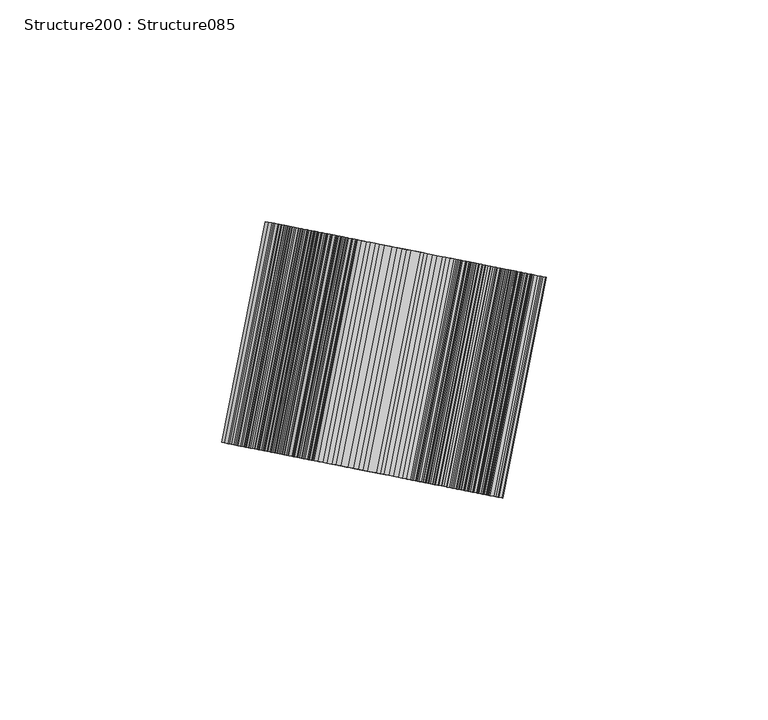
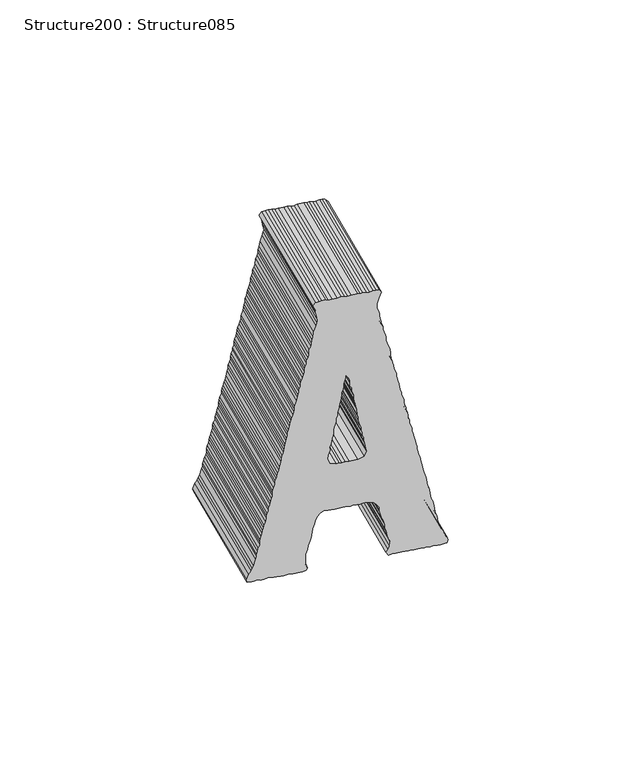
"""IFC4 building model written with IfcOpenShell, lengths in millimetres: proxy geometry, Structure200 : Structure085."""

import ifcopenshell
import ifcopenshell.guid

model = None  # the IFC model being written
_history = None  # IfcOwnerHistory: only IFC2X3 demands one
_inside = {}  # id of a spatial element -> (the spatial element, [elements in it])
_under = {}  # id of a project, library or spatial element -> (it, [spatial elements below it])
_declared = {}  # id of a project -> (the project, [libraries it declares])
_typed = {}  # id of a type object -> (the type object, [elements of that type])
_made_of = {}  # id of a material, layer set ... -> (it, [elements and type objects made of it])


def new_model(schema):
    """Start an empty IFC model of exactly this schema.

    Asked for "IFC4X3", IfcOpenShell would pick the latest addendum, in which some entities
    have other attributes; the version numbers below select the first issue.
    IFC2X3 requires an IfcOwnerHistory on every rooted entity: one is made here for all.
    """
    global model, _history
    if schema == "IFC4X3":
        model = ifcopenshell.file(schema_version=(4, 3, 0, 0))
    else:
        model = ifcopenshell.file(schema=schema)
    _inside.clear()
    _under.clear()
    _declared.clear()
    _typed.clear()
    _made_of.clear()
    _history = None
    if model.schema == "IFC2X3":
        org = make("IfcOrganization", Name="unknown")
        user = make(
            "IfcPersonAndOrganization",
            ThePerson=make("IfcPerson", FamilyName="unknown"),
            TheOrganization=org,
        )
        app = make(
            "IfcApplication",
            ApplicationDeveloper=org,
            Version="unknown",
            ApplicationFullName="unknown",
            ApplicationIdentifier="unknown",
        )
        _history = make(
            "IfcOwnerHistory",
            OwningUser=user,
            OwningApplication=app,
            ChangeAction="ADDED",
            CreationDate=0,
        )
    return model


def make(cls, **values):
    """One entity of the class cls with the attributes given. An attribute that is None is left unset."""
    return model.create_entity(
        cls, **{name: value for name, value in values.items() if value is not None}
    )


def rooted(cls, **values):
    """An entity with a GlobalId (a new one), such as an element, a storey or a relation."""
    return make(cls, GlobalId=ifcopenshell.guid.new(), OwnerHistory=_history, **values)


def si_unit(unit_type, name, prefix=None):
    """IfcSIUnit, for example si_unit("LENGTHUNIT", "METRE", prefix="MILLI")."""
    return make("IfcSIUnit", UnitType=unit_type, Prefix=prefix, Name=name)


def assignment(units):
    """IfcUnitAssignment: the units of a project."""
    return None if units is None else make("IfcUnitAssignment", Units=units)


def point(xyz):
    """IfcCartesianPoint."""
    return None if xyz is None else make("IfcCartesianPoint", Coordinates=xyz)


def direction(xyz):
    """IfcDirection."""
    return None if xyz is None else make("IfcDirection", DirectionRatios=xyz)


def frame(location, z_axis=None, x_axis=None):
    """IfcAxis2Placement3D, a coordinate frame: its origin and axes. An axis left out is left unset."""
    return make(
        "IfcAxis2Placement3D",
        Location=point(location),
        Axis=direction(z_axis),
        RefDirection=direction(x_axis),
    )


def origin():
    """The frame at (0, 0, 0) with its axes left unset."""
    return frame((0.0, 0.0, 0.0))


def place(relative_to, where):
    """IfcLocalPlacement: puts the frame where relative to a parent placement (None: the world)."""
    return make(
        "IfcLocalPlacement", PlacementRelTo=relative_to, RelativePlacement=where
    )


def context(
    kind, dimensions, precision=None, world=None, true_north=None, identifier=None
):
    """IfcGeometricRepresentationContext, for example the 3D "Model" context."""
    return make(
        "IfcGeometricRepresentationContext",
        ContextIdentifier=identifier,
        ContextType=kind,
        CoordinateSpaceDimension=dimensions,
        Precision=precision,
        WorldCoordinateSystem=world,
        TrueNorth=true_north,
    )


def project(units=None, contexts=None):
    """IfcProject with its units and contexts."""
    return rooted(
        "IfcProject",
        Name="project",
        RepresentationContexts=contexts,
        UnitsInContext=assignment(units),
    )


def spatial(cls, under=None, at=None, **own):
    """A site, building, storey or space (cls), placed at a placement, below another one or the project."""
    s = rooted(cls, ObjectPlacement=at, **own)
    if under is not None:
        _under.setdefault(under.id(), (under, []))[1].append(s)
    return s


def polyline(points):
    """IfcPolyline through the points."""
    return make("IfcPolyline", Points=[point(p) for p in points])


def outline(outer, holes=None, kind="AREA"):
    """IfcArbitraryClosedProfileDef: a profile drawn as a closed curve; with holes, ...WithVoids."""
    if holes is None:
        return make("IfcArbitraryClosedProfileDef", ProfileType=kind, OuterCurve=outer)
    return make(
        "IfcArbitraryProfileDefWithVoids",
        ProfileType=kind,
        OuterCurve=outer,
        InnerCurves=holes,
    )


def extrude(swept, where, along, depth):
    """IfcExtrudedAreaSolid: the profile swept, set in the frame where, extruded along a direction by depth."""
    return make(
        "IfcExtrudedAreaSolid",
        SweptArea=swept,
        Position=where,
        ExtrudedDirection=direction(along),
        Depth=depth,
    )


def shape(context_of_items, identifier, shape_type, items):
    """IfcShapeRepresentation: the items that make up one representation, for example the "Body"."""
    return make(
        "IfcShapeRepresentation",
        ContextOfItems=context_of_items,
        RepresentationIdentifier=identifier,
        RepresentationType=shape_type,
        Items=items,
    )


def source(mapping_origin, context_of_items, identifier, shape_type, items):
    """IfcRepresentationMap: a shape defined once, which mapped items show again and again."""
    return make(
        "IfcRepresentationMap",
        MappingOrigin=mapping_origin,
        MappedRepresentation=shape(context_of_items, identifier, shape_type, items),
    )


def transform(
    local_origin,
    x_axis=None,
    y_axis=None,
    z_axis=None,
    scale=None,
    scale2=None,
    scale3=None,
    uniform=True,
):
    """IfcCartesianTransformationOperator3D, or its non-uniform kind. x_axis, y_axis, z_axis: its Axis1, 2, 3."""
    if uniform:
        return make(
            "IfcCartesianTransformationOperator3D",
            Axis1=direction(x_axis),
            Axis2=direction(y_axis),
            LocalOrigin=point(local_origin),
            Scale=scale,
            Axis3=direction(z_axis),
        )
    return make(
        "IfcCartesianTransformationOperator3DnonUniform",
        Axis1=direction(x_axis),
        Axis2=direction(y_axis),
        LocalOrigin=point(local_origin),
        Scale=scale,
        Axis3=direction(z_axis),
        Scale2=scale2,
        Scale3=scale3,
    )


def mapped(mapping_source, mapping_target):
    """IfcMappedItem: shows the shape of a source again, moved by a transform."""
    return make(
        "IfcMappedItem", MappingSource=mapping_source, MappingTarget=mapping_target
    )


def made_of(thing, what):
    """Note that an element or type object is made of a material, layer set ...; save() writes the relation."""
    if what is not None:
        _made_of.setdefault(what.id(), (what, []))[1].append(thing)
    return thing


def element(
    cls,
    number,
    at=None,
    inside=None,
    cuts=None,
    type_object=None,
    material=None,
    context=None,
    identifier="Body",
    shape_type=None,
    held_by="IfcProductDefinitionShape",
    body=None,
    shapes=None,
    **own,
):
    """One element of the class cls, such as IfcWall. Its Tag is "e" and its number.

    at: its placement. inside: the storey or other place that contains it. cuts: it is an
    opening in that element (IfcRelVoidsElement). A single representation is given by context,
    identifier, shape_type and body (its items); several are given by shapes. held_by: the class
    of the entity that holds the representations. save() writes the other relations.
    """
    e = rooted(cls, Tag="e%d" % number, ObjectPlacement=at, **own)
    if body is not None:
        shapes = [shape(context, identifier, shape_type, body)]
    if shapes is not None:
        e.Representation = make(held_by, Representations=shapes)
    if inside is not None:
        _inside.setdefault(inside.id(), (inside, []))[1].append(e)
    if cuts is not None:
        rooted(
            "IfcRelVoidsElement", RelatingBuildingElement=cuts, RelatedOpeningElement=e
        )
    if type_object is not None:
        _typed.setdefault(type_object.id(), (type_object, []))[1].append(e)
    return made_of(e, material)


def aggregate(whole, parts):
    """IfcRelAggregates: a whole, such as a stair, and the parts it consists of."""
    return rooted("IfcRelAggregates", RelatingObject=whole, RelatedObjects=parts)


def save(model, path):
    """Write the relations noted so far, then the file.

    IfcRelAggregates (storeys below a building ...), IfcRelContainedInSpatialStructure (elements
    in a storey), IfcRelDefinesByType, IfcRelAssociatesMaterial and IfcRelDeclares: one each for
    every whole, place, type object, material and project.
    """
    for whole, parts in _under.values():
        aggregate(whole, parts)
    for where, things in _inside.values():
        rooted(
            "IfcRelContainedInSpatialStructure",
            RelatedElements=things,
            RelatingStructure=where,
        )
    for kind, things in _typed.values():
        rooted("IfcRelDefinesByType", RelatedObjects=things, RelatingType=kind)
    for what, things in _made_of.values():
        rooted("IfcRelAssociatesMaterial", RelatedObjects=things, RelatingMaterial=what)
    for by, libraries in _declared.values():
        rooted("IfcRelDeclares", RelatingContext=by, RelatedDefinitions=libraries)
    model.write(path)


def structure200_structure085_df85b049(model_context):
    return source(origin(), model_context, "Body", "SweptSolid", [
        extrude(outline(polyline([(0.9094651, 0.0), (2.0811665, -0.5237609), (2.9906316, -0.6522104), (4.1562841, -0.7856413), (5.1991801, -1.1709897), (5.9748585, -1.2994392), (7.1504738, -1.6901249), (8.1894559, -1.6901249), (9.3551083, -2.0804549), (10.2645735, -2.3423353), (11.4362748, -2.6042157), (12.3453841, -2.8611147), (13.3818755, -2.9895642), (14.1582655, -3.3802499), (15.4626861, -3.5086994), (16.3721513, -3.5086994), (17.5385154, -3.7705798), (19.491944, -4.4178087), (20.2718921, -4.6796891), (21.3101626, -4.9369439), (22.3470097, -4.9369439), (23.2561191, -5.1988244), (24.4278204, -5.5891542), (25.4700048, -5.9745027), (26.6363689, -5.9745027), (27.4124031, -6.3648326), (28.7175354, -6.6270689), (30.535754, -7.0173988), (31.5743802, -7.1508297), (32.7400327, -7.4077286), (33.6555467, -7.7980585), (35.4741211, -7.7980585), (36.5102567, -7.5411595), (37.5492387, -7.2792792), (38.3288311, -6.8889493), (39.3671015, -6.3648326), (40.4099976, -7.2792792), (40.5395145, -8.1883885), (40.5395145, -9.0978536), (40.2826155, -10.2691991), (40.2826155, -11.306758), (40.5395145, -12.4781034), (40.4099976, -13.2541377), (40.5395145, -14.1682284), (40.5395145, -16.2437018), (40.2826155, -17.2816164), (40.2826155, -18.319531), (40.5395145, -19.4905208), (40.4099976, -20.6618662), (40.4099976, -22.3519912), (40.2826155, -23.5183553), (40.5395145, -24.4274647), (40.5395145, -25.5988102), (40.4099976, -26.5082753), (40.2826155, -27.6742836), (39.2382962, -28.4552992), (38.3288311, -27.936164), (37.4197218, -27.6742836), (36.6397736, -27.5508155), (35.4741211, -27.2889351), (33.5199809, -26.8986051), (32.6112274, -27.1604856), (31.4448633, -27.4173846), (29.3636968, -28.1934188), (27.545834, -28.4552992), (26.5089869, -28.7171796), (25.3372855, -28.8456292), (24.2943895, -29.1075095), (23.2561191, -29.6262889), (21.3101626, -29.7550942), (20.2718921, -30.0169746), (19.491944, -30.5357541), (18.3202426, -30.5357541), (17.2816164, -30.9211026), (16.3721513, -31.1829829), (15.3356599, -31.1829829), (14.1582655, -31.4452191), (13.1253323, -31.835549), (12.2158672, -32.225879), (11.4362748, -32.3543285), (10.2645735, -32.4877594), (9.3551083, -32.8731079), (8.1894559, -32.8731079), (7.1504738, -33.2637935), (6.2374505, -33.392243), (5.0714422, -33.6541235), (3.2475306, -34.3013524), (2.0811665, -34.3013524), (1.1720572, -34.5632328), (0.1334309, -34.8204876), (-1.0382704, -35.3442485), (-1.8178628, -35.4726979), (-2.8568449, -35.7345783), (-3.8990293, -35.8630278), (-5.0653934, -36.2487321), (-5.8471206, -36.5106125), (-7.0166871, -36.5106125), (-8.1826954, -36.9009425), (-8.9644226, -37.0343734), (-10.1364798, -37.4247032), (-11.1690572, -37.5481713), (-12.2115974, -37.6766208), (-12.9915456, -37.938857), (-14.03373, -38.3291869), (-15.3292552, -38.4626179), (-16.3678815, -38.7195169), (-18.1861001, -39.1098468), (-19.3581573, -39.3667458), (-20.2672666, -39.7574314), (-21.4371888, -40.0193119), (-22.2189161, -40.2811923), (-23.1223323, -40.5430727), (-24.1648726, -40.5430727), (-25.465735, -41.0568707), (-26.5025822, -41.3191069), (-27.4173846, -41.4475564), (-28.4560108, -41.4475564), (-29.235959, -41.7094369), (-30.5311284, -42.0997667), (-31.3110766, -42.2282162), (-32.3536168, -42.6135647), (-33.5214042, -42.6135647), (-34.4308693, -43.1376814), (-35.3399786, -43.3995618), (-36.37647, -43.3995618), (-37.5424783, -43.6564608), (-38.7202285, -44.0467906), (-39.6236447, -44.3036896), (-40.405372, -44.5659258), (-41.5752942, -44.6943753), (-42.6139205, -45.0847053), (-43.7856218, -45.3465857), (-44.8221132, -45.3465857), (-45.7372714, -45.4800166), (-46.6406876, -45.9938146), (-47.812389, -46.2560508), (-48.8510152, -46.5179312), (-49.7601245, -46.5179312), (-50.6731478, -46.9082611), (-52.8777823, -47.5505086), (-53.7929405, -47.9461758), (-54.5689747, -48.3365056), (-55.738897, -49.1171654), (-57.5532016, -49.7647502), (-58.4665807, -49.5028697), (-58.5957419, -48.2030748), (-58.4665807, -47.4270405), (-58.3331498, -46.2560508), (-58.5957419, -45.2181362), (-58.5957419, -44.0467906), (-58.3331498, -43.0092319), (-58.3331498, -42.0997667), (-58.4665807, -41.0568707), (-58.4665807, -40.1477614), (-58.5957419, -38.8529478), (-58.5957419, -37.938857), (-58.4665807, -36.9009425), (-58.3331498, -35.7345783), (-58.5957419, -34.8204876), (-58.5957419, -31.835549), (-58.3331498, -30.6642036), (-57.4297336, -30.1454241), (-56.6480063, -30.5357541), (-55.6115149, -30.7976345), (-53.3972734, -30.7976345), (-52.3586471, -30.7976345), (-51.4495378, -30.5357541), (-50.6731478, -30.1454241), (-49.3683714, -30.0169746), (-48.4592621, -29.7550942), (-47.5497969, -29.3644085), (-46.6406876, -29.1075095), (-45.6038405, -28.8456292), (-43.2661308, -28.5887302), (-41.5752942, -27.936164), (-40.2762109, -27.6742836), (-38.9767716, -27.0270546), (-38.1950444, -26.1175896), (-37.4190102, -24.689345), (-37.6759092, -23.6517862), (-37.6759092, -21.5713314), (-37.5424783, -20.2715363), (-37.5424783, -17.5434968), (-37.6759092, -16.3721513), (-37.4190102, -15.463042), (-37.5424783, -14.4201459), (-37.6759092, -13.3825872), (-37.5424783, -12.4781034), (-37.4190102, -11.173327), (-37.6759092, -10.3976486), (-38.0676623, -8.8359732), (-38.8476105, -8.0549575), (-40.2762109, -7.0173988), (-41.4422191, -7.0173988), (-42.6139205, -6.7604998), (-44.561656, -6.2363831), (-45.3472973, -5.7225851), (-46.5133056, -5.4607047), (-47.2932538, -5.3322553), (-48.33188, -5.3322553), (-49.3683714, -4.8081386), (-50.4126907, -4.6796891), (-51.4495378, -4.5462582), (-52.3586471, -4.1609097), (-53.6595096, -3.7705798), (-55.3489229, -3.8990293), (-56.6480063, -4.2893592), (-57.2966585, -4.9369439), (-58.5957419, -4.1609097), (-58.4665807, -2.9895642), (-58.3331498, -1.9520054), (-58.3331498, 0.1288053), (-58.4665807, 1.166364), (-58.4665807, 2.2092601), (-58.3331498, 3.113388), (-58.4665807, 4.0228531), (-58.4665807, 5.3276296), (-58.3331498, 6.1033079), (-58.4665807, 7.403103), (-58.3331498, 8.1837628), (-58.5957419, 9.2216774), (-58.3331498, 10.3930229), (-58.5957419, 11.5593871), (-58.4665807, 12.4684963), (-58.3331498, 13.5113924), (-58.3331498, 14.5489512), (-57.2966585, 14.9396369), (-56.3875492, 14.6774007), (-55.738897, 14.0251904), (-54.5689747, 13.7732728), (-53.7929405, 13.3829429), (-52.6151903, 12.8588263), (-50.6731478, 11.9546984), (-49.8875066, 11.692818), (-48.5941162, 11.5593871), (-47.5497969, 11.3021323), (-46.6406876, 11.0402518), (-45.8646534, 10.6549034), (-44.561656, 10.5214724), (-42.6139205, 10.2645734), (-41.4422191, 9.8738877), (-40.5384471, 9.4835579), (-39.6236447, 9.2216774), (-38.4576364, 9.0882465), (-37.4190102, 8.9647784), (-36.5059869, 8.8363289), (-35.6004358, 8.3125681), (-34.2956593, 8.1837628), (-33.3922431, 8.0503318), (-32.3536168, 7.9218824), (-31.4405935, 7.5315524), (-30.4019673, 7.146204), (-29.235959, 6.8843236), (-27.5447666, 6.6224432), (-26.3752002, 6.2317574), (-25.203143, 6.1033079), (-24.4235506, 5.8414275), (-23.3849244, 5.4560791), (-22.4793732, 5.3276296), (-21.3037579, 4.9369439), (-20.2672666, 4.9369439), (-19.3581573, 4.6750635), (-18.319531, 4.413183), (-17.1474738, 4.1513026), (-15.2018732, 3.6375046), (-14.1632469, 3.3756242), (-13.1207067, 3.3756242), (-12.2115974, 2.9849385), (-11.3024881, 2.5946086), (-10.0012698, 2.5946086), (-9.2270147, 2.0808106), (-8.1826954, 2.0808106), (-7.0166871, 1.9473797), (-5.9745027, 1.4282445), (-5.0653934, 1.4282445), (-4.1619771, 0.9044837), (-2.8568449, 0.7760342), (-1.9473797, 0.7760342), (-0.7817273, 0.2572548), (0.0, 0.0), (0.9094651, 0.0)]), holes=[polyline([(-20.9137838, -13.9063479), (-20.9137838, -16.8912865), (-20.7903157, -18.0622762), (-21.0472147, -19.2336218), (-20.7903157, -20.1430869), (-20.9137838, -21.0472147), (-20.2672666, -22.9992201), (-18.5817672, -23.6517862), (-17.2809048, -23.3899058), (-16.3678815, -23.1280254), (-15.4623303, -22.8657892), (-14.1632469, -22.9992201), (-13.2480888, -22.4804408), (-12.2115974, -22.3519912), (-11.3024881, -22.2185603), (-10.393023, -21.8282304), (-9.3508386, -21.6997809), (-8.3122123, -21.6997809), (-7.146204, -21.5713314), (-6.3644768, -21.1806457), (-5.3276296, -20.9187652), (-4.2854452, -20.9187652), (-3.117302, -20.3999858), (-1.9473797, -20.3999858), (-1.0382704, -20.009656), (-0.2561874, -19.8812065), (1.0389821, -19.7477756), (2.0811665, -19.4905208), (3.1180136, -19.2336218), (4.0274787, -19.1051723), (5.0714422, -19.1051723), (6.1082894, -18.5814114), (7.0177545, -18.4529619), (8.1894559, -18.4529619), (9.2216774, -18.0622762), (10.1368356, -17.8003958), (11.0463007, -17.8003958), (10.1368356, -17.1531669), (9.0928721, -16.762837), (8.056025, -16.6343875), (6.8900167, -16.6343875), (6.1082894, -16.1102708), (4.9365881, -15.9818214), (3.1180136, -15.463042), (1.8189302, -15.3345925), (0.9094651, -15.206143), (0.0, -14.9442626), (-1.0382704, -14.8108317), (-2.2078369, -14.4201459), (-4.2854452, -14.2916964), (-5.3276296, -14.0347974), (-6.3644768, -13.9063479), (-8.1826954, -13.5160181), (-9.2270147, -12.9919014), (-10.2638619, -12.9919014), (-11.1690572, -12.7350024), (-12.3446725, -12.6065529), (-13.1207067, -12.216223), (-14.286715, -12.216223), (-15.4623303, -11.8258931), (-17.2809048, -11.5640128), (-18.5817672, -11.306758), (-20.1377496, -12.0877735), (-20.9137838, -13.9063479)])]), frame((-3026.1525446, 235069.0440944, 444.9951864), z_axis=(0.19466222296394123, 0.9808703374813295, 0.0), x_axis=(0.0, 0.0, 1.0)), (0.0, 0.0, 1.0), 50.8),
    ])


if __name__ == "__main__":
    model = new_model("IFC4")
    model_context = context("Model", 3, world=origin())
    ifc_project = project(units=[si_unit("LENGTHUNIT", "METRE", prefix="MILLI")], contexts=[model_context])
    site = spatial("IfcSite", under=ifc_project)
    building = spatial("IfcBuilding", under=site)
    placement = place(None, origin())
    structure200_structure085_shape = structure200_structure085_df85b049(model_context)
    element("IfcBuildingElementProxy", 1, Name="Structure200 : Structure085", ObjectType="Structure200 : Structure085", at=placement, inside=building, context=model_context, shape_type="MappedRepresentation", body=[
        mapped(structure200_structure085_shape, transform((0.0, 0.0, 0.0), x_axis=(1.0, 0.0, 0.0), y_axis=(0.0, 1.0, 0.0), z_axis=(0.0, 0.0, 1.0))),
    ])
    save(model, "model.ifc")

# Revit data of these elements
# Type "Structure200 : Structure085"
#   NameOverride = "Structure085"
# Element 1 (IfcBuildingElementProxy, "Structure200 : Structure085")
#   Materials on its faces: "BRUSHED ALUMINUM LETTERING"
# Materials
#   "BRUSHED ALUMINUM LETTERING": class "Unassigned", colour RGB 169 181 186, transparency 0, Cost = 0
